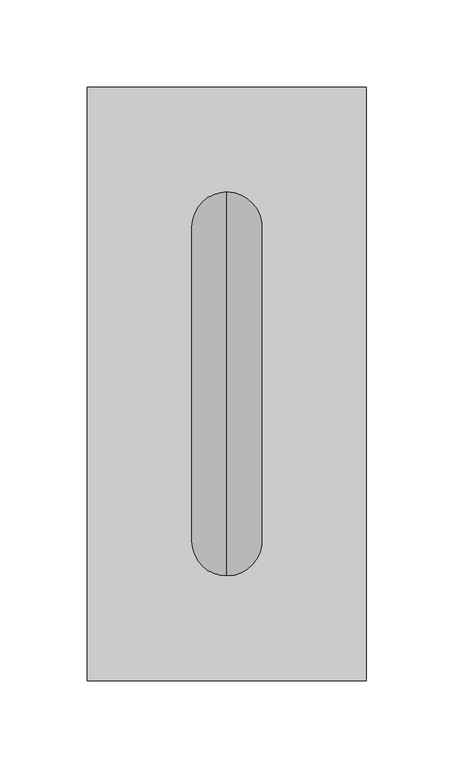
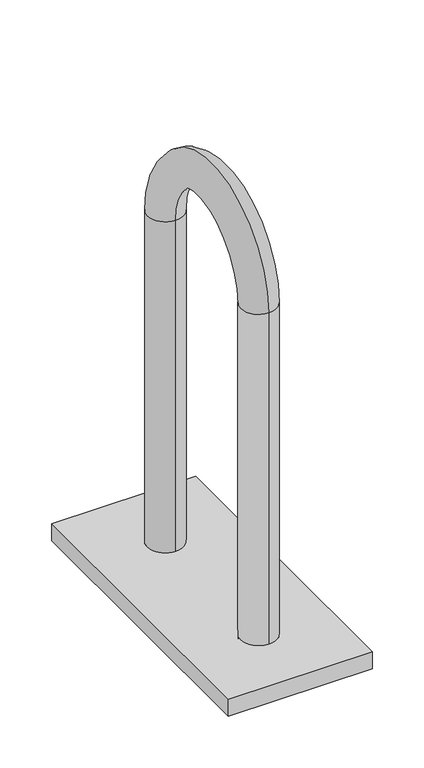
"""IFC4 building model written with IfcOpenShell, lengths in millimetres: proxy geometry, Опорный поручень : Опорный поручень для раковины."""

import ifcopenshell
import ifcopenshell.guid

model = None  # the IFC model being written
_history = None  # IfcOwnerHistory: only IFC2X3 demands one
_inside = {}  # id of a spatial element -> (the spatial element, [elements in it])
_under = {}  # id of a project, library or spatial element -> (it, [spatial elements below it])
_declared = {}  # id of a project -> (the project, [libraries it declares])
_typed = {}  # id of a type object -> (the type object, [elements of that type])
_made_of = {}  # id of a material, layer set ... -> (it, [elements and type objects made of it])


def new_model(schema):
    """Start an empty IFC model of exactly this schema.

    Asked for "IFC4X3", IfcOpenShell would pick the latest addendum, in which some entities
    have other attributes; the version numbers below select the first issue.
    IFC2X3 requires an IfcOwnerHistory on every rooted entity: one is made here for all.
    """
    global model, _history
    if schema == "IFC4X3":
        model = ifcopenshell.file(schema_version=(4, 3, 0, 0))
    else:
        model = ifcopenshell.file(schema=schema)
    _inside.clear()
    _under.clear()
    _declared.clear()
    _typed.clear()
    _made_of.clear()
    _history = None
    if model.schema == "IFC2X3":
        org = make("IfcOrganization", Name="unknown")
        user = make(
            "IfcPersonAndOrganization",
            ThePerson=make("IfcPerson", FamilyName="unknown"),
            TheOrganization=org,
        )
        app = make(
            "IfcApplication",
            ApplicationDeveloper=org,
            Version="unknown",
            ApplicationFullName="unknown",
            ApplicationIdentifier="unknown",
        )
        _history = make(
            "IfcOwnerHistory",
            OwningUser=user,
            OwningApplication=app,
            ChangeAction="ADDED",
            CreationDate=0,
        )
    return model


def make(cls, **values):
    """One entity of the class cls with the attributes given. An attribute that is None is left unset."""
    return model.create_entity(
        cls, **{name: value for name, value in values.items() if value is not None}
    )


def rooted(cls, **values):
    """An entity with a GlobalId (a new one), such as an element, a storey or a relation."""
    return make(cls, GlobalId=ifcopenshell.guid.new(), OwnerHistory=_history, **values)


def si_unit(unit_type, name, prefix=None):
    """IfcSIUnit, for example si_unit("LENGTHUNIT", "METRE", prefix="MILLI")."""
    return make("IfcSIUnit", UnitType=unit_type, Prefix=prefix, Name=name)


def assignment(units):
    """IfcUnitAssignment: the units of a project."""
    return None if units is None else make("IfcUnitAssignment", Units=units)


def point(xyz):
    """IfcCartesianPoint."""
    return None if xyz is None else make("IfcCartesianPoint", Coordinates=xyz)


def direction(xyz):
    """IfcDirection."""
    return None if xyz is None else make("IfcDirection", DirectionRatios=xyz)


def frame(location, z_axis=None, x_axis=None):
    """IfcAxis2Placement3D, a coordinate frame: its origin and axes. An axis left out is left unset."""
    return make(
        "IfcAxis2Placement3D",
        Location=point(location),
        Axis=direction(z_axis),
        RefDirection=direction(x_axis),
    )


def origin():
    """The frame at (0, 0, 0) with its axes left unset."""
    return frame((0.0, 0.0, 0.0))


def origin_with_axes():
    """The frame at (0, 0, 0) with the z axis (0, 0, 1) and the x axis (1, 0, 0) written out."""
    return frame((0.0, 0.0, 0.0), z_axis=(0.0, 0.0, 1.0), x_axis=(1.0, 0.0, 0.0))


def place(relative_to, where):
    """IfcLocalPlacement: puts the frame where relative to a parent placement (None: the world)."""
    return make(
        "IfcLocalPlacement", PlacementRelTo=relative_to, RelativePlacement=where
    )


def context(
    kind, dimensions, precision=None, world=None, true_north=None, identifier=None
):
    """IfcGeometricRepresentationContext, for example the 3D "Model" context."""
    return make(
        "IfcGeometricRepresentationContext",
        ContextIdentifier=identifier,
        ContextType=kind,
        CoordinateSpaceDimension=dimensions,
        Precision=precision,
        WorldCoordinateSystem=world,
        TrueNorth=true_north,
    )


def project(units=None, contexts=None):
    """IfcProject with its units and contexts."""
    return rooted(
        "IfcProject",
        Name="project",
        RepresentationContexts=contexts,
        UnitsInContext=assignment(units),
    )


def spatial(cls, under=None, at=None, **own):
    """A site, building, storey or space (cls), placed at a placement, below another one or the project."""
    s = rooted(cls, ObjectPlacement=at, **own)
    if under is not None:
        _under.setdefault(under.id(), (under, []))[1].append(s)
    return s


def polyline(points):
    """IfcPolyline through the points."""
    return make("IfcPolyline", Points=[point(p) for p in points])


def circle_curve(where, radius):
    """IfcCircle in the frame where."""
    return make("IfcCircle", Position=where, Radius=radius)


def ellipse_curve(where, semi_axis1, semi_axis2):
    """IfcEllipse in the frame where."""
    return make(
        "IfcEllipse", Position=where, SemiAxis1=semi_axis1, SemiAxis2=semi_axis2
    )


def trimmed(basis, trim1, trim2, sense, master):
    """IfcTrimmedCurve: the piece of a basis curve between two trims."""
    return make(
        "IfcTrimmedCurve",
        BasisCurve=basis,
        Trim1=trim1,
        Trim2=trim2,
        SenseAgreement=sense,
        MasterRepresentation=master,
    )


def outline(outer, holes=None, kind="AREA"):
    """IfcArbitraryClosedProfileDef: a profile drawn as a closed curve; with holes, ...WithVoids."""
    if holes is None:
        return make("IfcArbitraryClosedProfileDef", ProfileType=kind, OuterCurve=outer)
    return make(
        "IfcArbitraryProfileDefWithVoids",
        ProfileType=kind,
        OuterCurve=outer,
        InnerCurves=holes,
    )


def extrude(swept, where, along, depth):
    """IfcExtrudedAreaSolid: the profile swept, set in the frame where, extruded along a direction by depth."""
    return make(
        "IfcExtrudedAreaSolid",
        SweptArea=swept,
        Position=where,
        ExtrudedDirection=direction(along),
        Depth=depth,
    )


def shape(context_of_items, identifier, shape_type, items):
    """IfcShapeRepresentation: the items that make up one representation, for example the "Body"."""
    return make(
        "IfcShapeRepresentation",
        ContextOfItems=context_of_items,
        RepresentationIdentifier=identifier,
        RepresentationType=shape_type,
        Items=items,
    )


def source(mapping_origin, context_of_items, identifier, shape_type, items):
    """IfcRepresentationMap: a shape defined once, which mapped items show again and again."""
    return make(
        "IfcRepresentationMap",
        MappingOrigin=mapping_origin,
        MappedRepresentation=shape(context_of_items, identifier, shape_type, items),
    )


def transform(
    local_origin,
    x_axis=None,
    y_axis=None,
    z_axis=None,
    scale=None,
    scale2=None,
    scale3=None,
    uniform=True,
):
    """IfcCartesianTransformationOperator3D, or its non-uniform kind. x_axis, y_axis, z_axis: its Axis1, 2, 3."""
    if uniform:
        return make(
            "IfcCartesianTransformationOperator3D",
            Axis1=direction(x_axis),
            Axis2=direction(y_axis),
            LocalOrigin=point(local_origin),
            Scale=scale,
            Axis3=direction(z_axis),
        )
    return make(
        "IfcCartesianTransformationOperator3DnonUniform",
        Axis1=direction(x_axis),
        Axis2=direction(y_axis),
        LocalOrigin=point(local_origin),
        Scale=scale,
        Axis3=direction(z_axis),
        Scale2=scale2,
        Scale3=scale3,
    )


def mapped(mapping_source, mapping_target):
    """IfcMappedItem: shows the shape of a source again, moved by a transform."""
    return make(
        "IfcMappedItem", MappingSource=mapping_source, MappingTarget=mapping_target
    )


def made_of(thing, what):
    """Note that an element or type object is made of a material, layer set ...; save() writes the relation."""
    if what is not None:
        _made_of.setdefault(what.id(), (what, []))[1].append(thing)
    return thing


def element(
    cls,
    number,
    at=None,
    inside=None,
    cuts=None,
    type_object=None,
    material=None,
    context=None,
    identifier="Body",
    shape_type=None,
    held_by="IfcProductDefinitionShape",
    body=None,
    shapes=None,
    **own,
):
    """One element of the class cls, such as IfcWall. Its Tag is "e" and its number.

    at: its placement. inside: the storey or other place that contains it. cuts: it is an
    opening in that element (IfcRelVoidsElement). A single representation is given by context,
    identifier, shape_type and body (its items); several are given by shapes. held_by: the class
    of the entity that holds the representations. save() writes the other relations.
    """
    e = rooted(cls, Tag="e%d" % number, ObjectPlacement=at, **own)
    if body is not None:
        shapes = [shape(context, identifier, shape_type, body)]
    if shapes is not None:
        e.Representation = make(held_by, Representations=shapes)
    if inside is not None:
        _inside.setdefault(inside.id(), (inside, []))[1].append(e)
    if cuts is not None:
        rooted(
            "IfcRelVoidsElement", RelatingBuildingElement=cuts, RelatedOpeningElement=e
        )
    if type_object is not None:
        _typed.setdefault(type_object.id(), (type_object, []))[1].append(e)
    return made_of(e, material)


def aggregate(whole, parts):
    """IfcRelAggregates: a whole, such as a stair, and the parts it consists of."""
    return rooted("IfcRelAggregates", RelatingObject=whole, RelatedObjects=parts)


def save(model, path):
    """Write the relations noted so far, then the file.

    IfcRelAggregates (storeys below a building ...), IfcRelContainedInSpatialStructure (elements
    in a storey), IfcRelDefinesByType, IfcRelAssociatesMaterial and IfcRelDeclares: one each for
    every whole, place, type object, material and project.
    """
    for whole, parts in _under.values():
        aggregate(whole, parts)
    for where, things in _inside.values():
        rooted(
            "IfcRelContainedInSpatialStructure",
            RelatedElements=things,
            RelatingStructure=where,
        )
    for kind, things in _typed.values():
        rooted("IfcRelDefinesByType", RelatedObjects=things, RelatingType=kind)
    for what, things in _made_of.values():
        rooted("IfcRelAssociatesMaterial", RelatedObjects=things, RelatingMaterial=what)
    for by, libraries in _declared.values():
        rooted("IfcRelDeclares", RelatingContext=by, RelatedDefinitions=libraries)
    model.write(path)


def plane_surface(at):
    """IfcPlane: the flat surface through the origin of the frame at, square to its z axis."""
    return make("IfcPlane", Position=at)


def cylinder_surface(at, radius):
    """IfcCylindricalSurface: all points at the distance radius from the z axis of the frame at."""
    return make("IfcCylindricalSurface", Position=at, Radius=radius)


def revolved_surface(curve, axis_point, axis_direction):
    """IfcSurfaceOfRevolution: the curve turned about the line through axis_point along axis_direction."""
    return make(
        "IfcSurfaceOfRevolution",
        SweptCurve=make("IfcArbitraryOpenProfileDef", ProfileType="CURVE", Curve=curve),
        AxisPosition=make("IfcAxis1Placement", Location=point(axis_point), Axis=direction(axis_direction)),
    )


def advanced_brep(points, edges, surfaces, faces):
    """IfcAdvancedBrep: a solid bounded by faces that lie on surfaces and meet in shared edges.

    An edge is (start, end): straight between two places in points (the first is 0);
    or (start, end, curve); or (start, end, curve, False) where it runs against its curve.
    A face is (place in surfaces, loops), or (place, loops, False) where it looks against
    its surface's normal. A loop lists edges by number (the first is 1), with a minus sign
    where the edge is run from its end to its start. The first loop is the outer one.
    """
    corners = [point(p) for p in points]
    vertices = [make("IfcVertexPoint", VertexGeometry=c) for c in corners]
    made = []
    for start, end, *more in edges:
        made.append(
            make(
                "IfcEdgeCurve",
                EdgeStart=vertices[start],
                EdgeEnd=vertices[end],
                EdgeGeometry=more[0] if more else make("IfcPolyline", Points=[corners[start], corners[end]]),
                SameSense=more[1] if len(more) > 1 else True,
            )
        )
    hull = []
    for where, loops, *sense in faces:
        bounds = []
        for j, loop in enumerate(loops):
            ring = [make("IfcOrientedEdge", EdgeElement=made[abs(k) - 1], Orientation=k > 0) for k in loop]
            bounds.append(
                make(
                    "IfcFaceOuterBound" if j == 0 else "IfcFaceBound",
                    Bound=make("IfcEdgeLoop", EdgeList=ring),
                    Orientation=True,
                )
            )
        hull.append(make("IfcAdvancedFace", Bounds=bounds, FaceSurface=surfaces[where], SameSense=sense[0] if sense else True))
    return make("IfcAdvancedBrep", Outer=make("IfcClosedShell", CfsFaces=hull))


def mechanical_equipment_f31a89b7(model_context):
    return source(origin(), model_context, "Body", "SolidModel", [
        extrude(outline(polyline([(80.0, -170.0), (-80.0, -170.0), (-80.0, 170.0), (80.0, 170.0), (80.0, -170.0)])), origin_with_axes(), (0.0, 0.0, 1.0), 20.0),
        advanced_brep(
        [(0.0, -110.0, 0.0), (0.0, -70.0, 0.0), (0.0, -70.0, 410.0), (0.0, -110.0, 410.0), (0.0, 70.0, 410.0), (0.0, 110.0, 410.0), (0.0, 110.0, 0.0), (0.0, 70.0, 0.0)],
        [
            (0, 1, circle_curve(frame((0.0, -90.0, 0.0), z_axis=(0.0, 0.0, -1.0), x_axis=(0.0, 1.0, 0.0)), 20.0)),
            (1, 0, circle_curve(frame((0.0, -90.0, 0.0), z_axis=(0.0, 0.0, -1.0), x_axis=(0.0, 1.0, 0.0)), 20.0)),
            (1, 2),
            (2, 3, circle_curve(frame((0.0, -90.0, 410.0), z_axis=(0.0, 0.0, -1.0), x_axis=(0.0, 1.0, 0.0)), 20.0)),
            (3, 0),
            (3, 2, circle_curve(frame((0.0, -90.0, 410.0), z_axis=(0.0, 0.0, -1.0), x_axis=(0.0, 1.0, 0.0)), 20.0)),
            (4, 5, circle_curve(frame((0.0, 90.0, 410.0), z_axis=(0.0, 0.0, 1.0), x_axis=(0.0, -1.0, 0.0)), 20.0)),
            (5, 3, circle_curve(frame((0.0, 0.0, 410.0), z_axis=(1.0, 0.0, 0.0), x_axis=(0.0, -1.0, 0.0)), 110.0)),
            (2, 4, circle_curve(frame((0.0, 0.0, 410.0), z_axis=(-1.0, 0.0, 0.0), x_axis=(0.0, -1.0, 0.0)), 70.0)),
            (5, 4, circle_curve(frame((0.0, 90.0, 410.0), z_axis=(0.0, 0.0, 1.0), x_axis=(0.0, -1.0, 0.0)), 20.0)),
            (6, 7, circle_curve(frame((0.0, 90.0, 0.0), z_axis=(0.0, 0.0, -1.0), x_axis=(0.0, -1.0, 0.0)), 20.0)),
            (7, 6, circle_curve(frame((0.0, 90.0, 0.0), z_axis=(0.0, 0.0, -1.0), x_axis=(0.0, -1.0, 0.0)), 20.0)),
            (4, 7),
            (6, 5),
        ],
        [
            plane_surface(frame((0.0, -90.0, 0.0), z_axis=(0.0, 0.0, -1.0), x_axis=(1.0, 0.0, 0.0))),
            cylinder_surface(frame((0.0, -90.0, 0.0), z_axis=(0.0, 0.0, -1.0), x_axis=(0.0, 1.0, 0.0)), 20.0),
            revolved_surface(trimmed(ellipse_curve(frame((0.0, -90.0, 410.0), z_axis=(0.0, 0.0, 1.0), x_axis=(0.0, 1.0, 0.0)), 20.0, 20.0), [point((0.0, -110.0, 410.0))], [point((0.0, -70.0, 410.0))], True, "CARTESIAN"), (0.0, 0.0, 410.0), (1.0, 0.0, 0.0)),
            revolved_surface(trimmed(ellipse_curve(frame((0.0, -90.0, 410.0), z_axis=(0.0, 0.0, 1.0), x_axis=(0.0, 1.0, 0.0)), 20.0, 20.0), [point((0.0, -70.0, 410.0))], [point((0.0, -110.0, 410.0))], True, "CARTESIAN"), (0.0, 0.0, 410.0), (1.0, 0.0, 0.0)),
            plane_surface(frame((0.0, 90.0, 0.0), z_axis=(0.0, 0.0, -1.0), x_axis=(1.0, 0.0, 0.0))),
            cylinder_surface(frame((0.0, 90.0, 410.0), z_axis=(0.0, 0.0, 1.0), x_axis=(0.0, -1.0, 0.0)), 20.0),
        ],
        [
            (0, [[1, 2]]),
            (1, [[3, 4, 5, -2]]),
            (1, [[-5, 6, -3, -1]]),
            (2, [[7, 8, -4, 9]]),
            (3, [[10, -9, -6, -8]]),
            (4, [[11, 12]]),
            (5, [[13, -11, 14, -7]]),
            (5, [[-14, -12, -13, -10]]),
        ],
    ),
    ])


if __name__ == "__main__":
    model = new_model("IFC4")
    model_context = context("Model", 3, world=origin())
    ifc_project = project(units=[si_unit("LENGTHUNIT", "METRE", prefix="MILLI")], contexts=[model_context])
    site = spatial("IfcSite", under=ifc_project)
    building = spatial("IfcBuilding", under=site)
    placement = place(None, origin())
    mechanical_equipment_shape = mechanical_equipment_f31a89b7(model_context)
    element("IfcBuildingElementProxy", 1, Name="Опорный поручень : Опорный поручень для раковины", ObjectType="Опорный поручень : Опорный поручень для раковины", at=placement, inside=building, context=model_context, shape_type="MappedRepresentation", body=[
        mapped(mechanical_equipment_shape, transform((0.0, 0.0, 0.0), x_axis=(1.0, 0.0, 0.0), y_axis=(0.0, 1.0, 0.0), z_axis=(0.0, 0.0, 1.0))),
    ])
    save(model, "model.ifc")

# Revit data of these elements
# Type "Опорный поручень : Опорный поручень для раковины"
#   Model = "МГН"
#   Default Elevation = 1219.2 mm
#   ADSK_Размер_Длина = 500 mm
#   ADSK_Размер_Диаметр = 40 mm
#   ADSK_Размер_Высота = 180 mm
#   Откидной = no
#   ADSK_Материал = Сталь, нержавеющая, полированная
# Element 1 (IfcBuildingElementProxy, "Опорный поручень : Опорный поручень для раковины")
#   Materials on its faces: "Сталь, нержавеющая, полированная"
# Materials
#   "Сталь, нержавеющая, полированная": class "Металл", colour RGB 120 120 120, transparency 0, Description = "Сталь нержавеющая 18/8, полированная", Cost = 0
